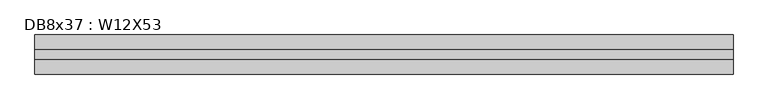
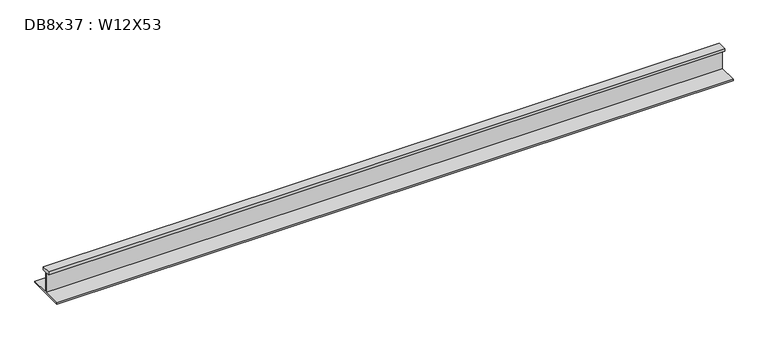
"""IFC4 building model written with IfcOpenShell, lengths in millimetres: beam geometry, DB8x37 : W12X53."""

from ifc_helpers import new_model, si_unit, frame, origin, place, context, project, spatial, polyline, outline, extrude, source, transform, mapped, element, save


def db8x37_w12x53_00467009(model_context):
    return source(origin(), model_context, "Body", "SweptSolid", [
        extrude(outline(polyline([(38.1, 145.415), (38.1, 120.015), (2.921, 120.015), (2.921, -48.4505), (152.4, -48.4505), (152.4, -58.1025), (-152.4, -58.1025), (-152.4, -48.4505), (-2.921, -48.4505), (-2.921, 120.015), (-38.1, 120.015), (-38.1, 145.415), (38.1, 145.415)])), frame((-2731.008, 0.0, 0.0), z_axis=(1.0, 0.0, 0.0), x_axis=(0.0, 1.0, 0.0)), (0.0, 0.0, 1.0), 5436.108),
    ])


if __name__ == "__main__":
    model = new_model("IFC4")
    model_context = context("Model", 3, world=origin())
    ifc_project = project(units=[si_unit("LENGTHUNIT", "METRE", prefix="MILLI")], contexts=[model_context])
    site = spatial("IfcSite", under=ifc_project)
    building = spatial("IfcBuilding", under=site)
    placement = place(None, origin())
    db8x37_w12x53_shape = db8x37_w12x53_00467009(model_context)
    element("IfcBeam", 1, ObjectType="DB8x37 : W12X53", at=placement, inside=building, context=model_context, shape_type="MappedRepresentation", body=[
        mapped(db8x37_w12x53_shape, transform((0.0, 0.0, 0.0), x_axis=(1.0, 0.0, 0.0), y_axis=(0.0, 1.0, 0.0), z_axis=(0.0, 0.0, 1.0))),
    ])
    save(model, "model.ifc")

# Revit data of these elements
# Type "DB8x37 : W12X53"
#   Assembly Code = "B10"
#   W = 53
#   Length [instance default] = 5' - 0"
#   bf = 0' - 10"
#   d = 1' - 0.1"
#   k = 0' - 1 3/8"
#   k2 = 0' - 0.8"
#   tf = 0' - 0.575"
#   tw = 0' - 0.345"
#   A = 0.108333 SF
#   Structural Material [instance default] = Steel ASTM A992
# Element 1 (IfcBeam, "DB8x37 : W12X53")
#   Materials on its faces: "Steel ASTM A992"
# Materials
#   "Steel ASTM A992": class "Metal", colour RGB 199 199 199, transparency 0, Description = "Structural steel 50ksi", Cost = 0
